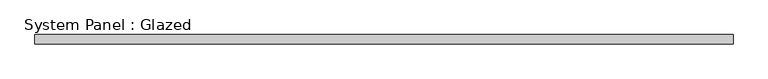
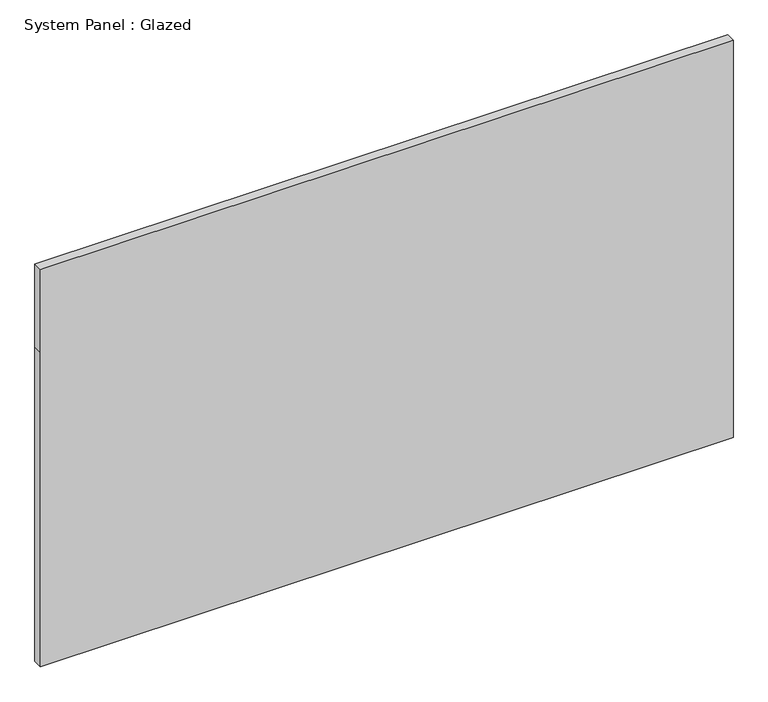
"""IFC4 building model written with IfcOpenShell, lengths in millimetres: plate geometry, System Panel : Glazed."""

from ifc_helpers import new_model, si_unit, frame, origin, place, context, project, spatial, polyline, outline, extrude, source, transform, mapped, element, save


def system_panel_glazed_56110c51(model_context):
    return source(origin(), model_context, "Body", "SweptSolid", [
        extrude(outline(polyline([(0.0, -952.5), (0.0, 952.5), (914.4, 952.5), (1155.7, 952.5), (1155.7, -952.5), (914.4, -952.5), (0.0, -952.5)])), frame((0.0, 19.05, 0.0), z_axis=(0.0, 1.0, 0.0), x_axis=(0.0, 0.0, 1.0)), (0.0, 0.0, 1.0), 25.4),
    ])


if __name__ == "__main__":
    model = new_model("IFC4")
    model_context = context("Model", 3, world=origin())
    ifc_project = project(units=[si_unit("LENGTHUNIT", "METRE", prefix="MILLI")], contexts=[model_context])
    site = spatial("IfcSite", under=ifc_project)
    building = spatial("IfcBuilding", under=site)
    placement = place(None, origin())
    system_panel_glazed_shape = system_panel_glazed_56110c51(model_context)
    element("IfcPlate", 1, ObjectType="System Panel : Glazed", at=placement, inside=building, context=model_context, shape_type="MappedRepresentation", body=[
        mapped(system_panel_glazed_shape, transform((0.0, 0.0, 0.0), x_axis=(1.0, 0.0, 0.0), y_axis=(0.0, 1.0, 0.0), z_axis=(0.0, 0.0, 1.0))),
    ])
    save(model, "model.ifc")

# Revit data of these elements
# Element 1 (IfcPlate, "System Panel : Glazed")
#   Materials on its faces: "Glass"
# Materials
#   "Glass": class "Glass", colour RGB 0 128 192, transparency 0.75
